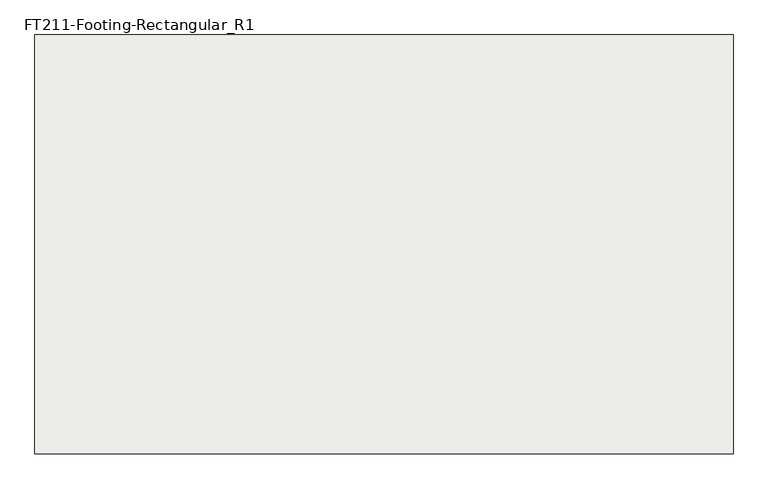
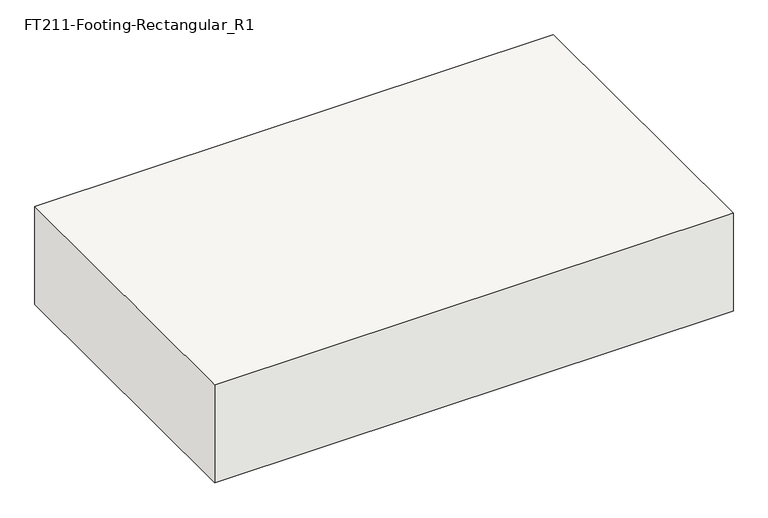
"""IFC4 building model written with IfcOpenShell, lengths in millimetres: slab geometry, FT211-Footing-Rectangular_R1 : H_SF_ACF_W2500xL1500xT500_Bitumen."""

from ifc_helpers import new_model, si_unit, frame, origin, place, context, project, spatial, polyline, outline, extrude, source, transform, mapped, element, save


def ft211_footing_rectangular_r1_907a7f09(model_context):
    return source(origin(), model_context, "Body", "SweptSolid", [
        extrude(outline(polyline([(1250.0, 750.0), (1250.0, -750.0), (-1250.0, -750.0), (-1250.0, 750.0), (1250.0, 750.0)])), frame((0.0, 0.0, -500.0), z_axis=(0.0, 0.0, 1.0), x_axis=(1.0, 0.0, 0.0)), (0.0, 0.0, 1.0), 500.0),
    ])


if __name__ == "__main__":
    model = new_model("IFC4")
    model_context = context("Model", 3, world=origin())
    ifc_project = project(units=[si_unit("LENGTHUNIT", "METRE", prefix="MILLI")], contexts=[model_context])
    site = spatial("IfcSite", under=ifc_project)
    building = spatial("IfcBuilding", under=site)
    placement = place(None, origin())
    ft211_footing_rectangular_r1_shape = ft211_footing_rectangular_r1_907a7f09(model_context)
    element("IfcSlab", 1, ObjectType="FT211-Footing-Rectangular_R1 : H_SF_ACF_W2500xL1500xT500_Bitumen", at=placement, inside=building, context=model_context, shape_type="MappedRepresentation", body=[
        mapped(ft211_footing_rectangular_r1_shape, transform((0.0, 0.0, 0.0), x_axis=(1.0, 0.0, 0.0), y_axis=(0.0, 1.0, 0.0), z_axis=(0.0, 0.0, 1.0))),
    ])
    save(model, "model.ifc")

# Revit data of these elements
# Type "FT211-Footing-Rectangular_R1 : H_SF_ACF_W2500xL1500xT500_Bitumen"
#   Top bar = "D25@300"
#   Description = "UG Shallow Foundation"
#   Bottom bar = "D20@300"
#   Width = 2500.000 mm
#   Length = 1500.000 mm
#   Foundation Thickness = 500.000 mm
#   Structural Material [instance default] = none
#   Assembly Code = ""
